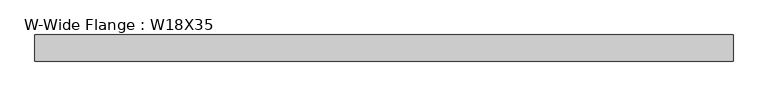
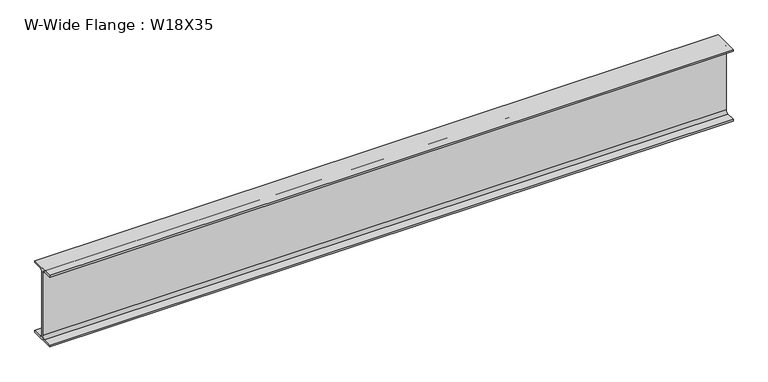
"""IFC4 building model written with IfcOpenShell, lengths in millimetres: beam geometry, W-Wide Flange : W18X35."""

from ifc_helpers import new_model, si_unit, point, frame, frame_2d, origin, place, context, project, spatial, polyline, circle_curve, trimmed, segment, composite_curve, outline, extrude, source, transform, mapped, element, save


def w_wide_flange_w18x35_de695320(model_context):
    return source(origin(), model_context, "Body", "SweptSolid", [
        extrude(outline(composite_curve([segment(polyline([(76.2, -213.995), (76.2, -224.79), (-76.2, -224.79), (-76.2, -213.995), (-21.59, -213.995)]), True, "CONTINUOUS"), segment(trimmed(circle_curve(frame_2d((-21.59, -196.215)), 17.78), [point((-21.59, -213.995))], [point((-3.81, -196.215))], True, "CARTESIAN"), True, "CONTINUOUS"), segment(polyline([(-3.81, -196.215), (-3.81, 196.215)]), True, "CONTINUOUS"), segment(trimmed(circle_curve(frame_2d((-21.59, 196.215)), 17.78), [point((-3.81, 196.215))], [point((-21.59, 213.995))], True, "CARTESIAN"), True, "CONTINUOUS"), segment(polyline([(-21.59, 213.995), (-76.2, 213.995), (-76.2, 224.79), (76.2, 224.79), (76.2, 213.995), (21.59, 213.995)]), True, "CONTINUOUS"), segment(trimmed(circle_curve(frame_2d((21.59, 196.215)), 17.78), [point((21.59, 213.995))], [point((3.81, 196.215))], True, "CARTESIAN"), True, "CONTINUOUS"), segment(polyline([(3.81, 196.215), (3.81, -196.215)]), True, "CONTINUOUS"), segment(trimmed(circle_curve(frame_2d((21.59, -196.215)), 17.78), [point((3.81, -196.215))], [point((21.59, -213.995))], True, "CARTESIAN"), True, "CONTINUOUS"), segment(polyline([(21.59, -213.995), (76.2, -213.995)]), True, "CONTINUOUS")], self_intersect=False)), frame((-2133.467846, 0.0, 0.0), z_axis=(1.0, 0.0, 0.0), x_axis=(0.0, 1.0, 0.0)), (0.0, 0.0, 1.0), 4067.545692),
    ])


if __name__ == "__main__":
    model = new_model("IFC4")
    model_context = context("Model", 3, world=origin())
    ifc_project = project(units=[si_unit("LENGTHUNIT", "METRE", prefix="MILLI")], contexts=[model_context])
    site = spatial("IfcSite", under=ifc_project)
    building = spatial("IfcBuilding", under=site)
    placement = place(None, origin())
    w_wide_flange_w18x35_shape = w_wide_flange_w18x35_de695320(model_context)
    element("IfcBeam", 1, ObjectType="W-Wide Flange : W18X35", at=placement, inside=building, context=model_context, shape_type="MappedRepresentation", body=[
        mapped(w_wide_flange_w18x35_shape, transform((0.0, 0.0, 0.0), x_axis=(1.0, 0.0, 0.0), y_axis=(0.0, 1.0, 0.0), z_axis=(0.0, 0.0, 1.0))),
    ])
    save(model, "model.ifc")

# Revit data of these elements
# Type "W-Wide Flange : W18X35"
#   Assembly Code = "B10"
#   W = 35
#   Start Extension Calculation [instance default] = 10' - 0"
#   Start Extension [instance default] = -0' - 0 1/2"
#   End Extension Calculation [instance default] = 10' - 0"
#   End Extension [instance default] = -0' - 0 1/2"
#   Length [instance default] = 5' - 0"
#   bf = 0' - 6"
#   d = 1' - 5.7"
#   k = 0' - 1 1/8"
#   k2 = 0' - 0.7"
#   tf = 0' - 0.425"
#   tw = 0' - 0.3"
#   A = 0.0715278 SF
#   Beam Material [instance default] = Metal - Steel - ASTM A992
# Element 1 (IfcBeam, "W-Wide Flange : W18X35")
#   Materials on its faces: "Metal - Steel - ASTM A992"
# Materials
#   "Metal - Steel - ASTM A992": class "Metal", colour RGB 128 0 0, transparency 0
